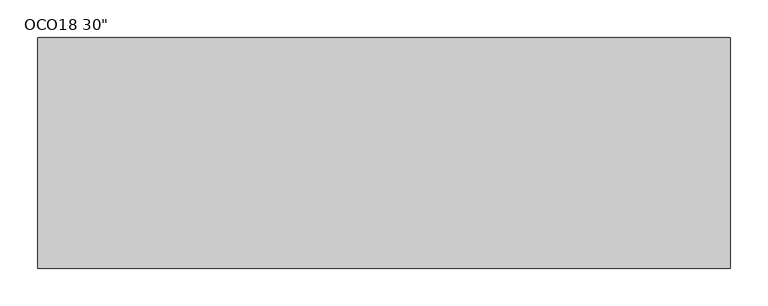
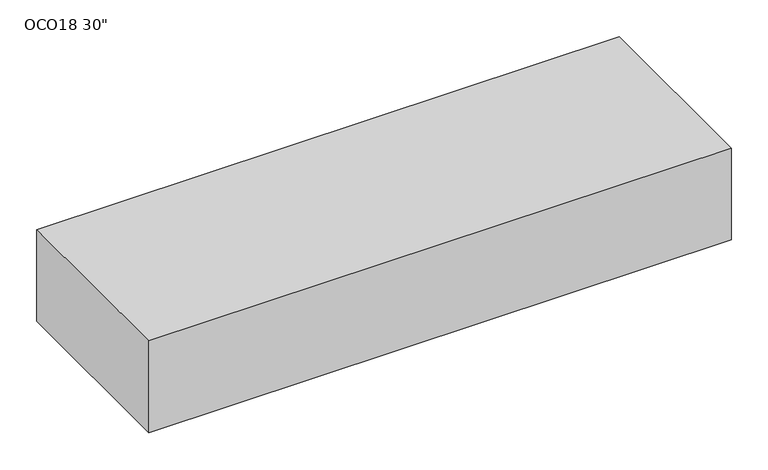
"""IFC4 building model written with IfcOpenShell, lengths in millimetres: furniture geometry."""

from ifc_helpers import new_model, si_unit, frame, origin, place, context, project, spatial, polyline, outline, extrude, faceted_brep, source, transform, mapped, element, save


def furniture_e9fbd180(model_context):
    return source(origin(), model_context, "Body", "SolidModel", [
        extrude(outline(polyline([(-125.8038372, 383.9486578), (-113.1038372, 383.9486578), (-113.1038372, 99.9612557), (-125.8038372, 99.9612557), (-125.8038372, 383.9486578)])), frame((0.0, 0.0, 1990.725), z_axis=(0.0, 0.0, 1.0), x_axis=(1.0, 0.0, 0.0)), (0.0, 0.0, 1.0), 133.35),
        extrude(outline(polyline([(172.6461628, 383.9486578), (185.3461628, 383.9486578), (185.3461628, 99.9612557), (172.6461628, 99.9612557), (172.6461628, 383.9486578)])), frame((0.0, 0.0, 1990.725), z_axis=(0.0, 0.0, 1.0), x_axis=(1.0, 0.0, 0.0)), (0.0, 0.0, 1.0), 133.35),
        extrude(outline(polyline([(-424.2538372, 383.9486578), (-411.5538372, 383.9486578), (-411.5538372, 99.9612557), (-424.2538372, 99.9612557), (-424.2538372, 383.9486578)])), frame((0.0, 0.0, 1990.725), z_axis=(0.0, 0.0, 1.0), x_axis=(1.0, 0.0, 0.0)), (0.0, 0.0, 1.0), 133.35),
        extrude(outline(polyline([(471.0961628, 383.9486578), (483.7961628, 383.9486578), (483.7961628, 99.9612557), (471.0961628, 99.9612557), (471.0961628, 383.9486578)])), frame((0.0, 0.0, 1990.725), z_axis=(0.0, 0.0, 1.0), x_axis=(1.0, 0.0, 0.0)), (0.0, 0.0, 1.0), 133.35),
        faceted_brep([(486.9711628, 385.7625, 1981.2), (-427.4288372, 385.7625, 1981.2), (-427.4288372, 385.7625, 2133.6), (486.9711628, 385.7625, 2133.6), (471.0961628, 385.7625, 1990.725), (471.0961628, 385.7625, 2124.075), (-411.5538372, 385.7625, 2124.075), (-411.5538372, 385.7625, 1990.725), (486.9711628, 80.9625, 1981.2), (486.9711628, 80.9625, 2133.6), (-427.4288372, 80.9625, 2133.6), (-427.4288372, 80.9625, 1981.2), (471.0961628, 99.9612557, 1990.725), (-411.5538372, 99.9612557, 1990.725), (-411.5538372, 99.9612557, 2124.075), (471.0961628, 99.9612557, 2124.075)], [[[0, 1, 2, 3], [4, 5, 6, 7]], [[8, 9, 10, 11]], [[1, 0, 8, 11]], [[2, 1, 11, 10]], [[3, 2, 10, 9]], [[0, 3, 9, 8]], [[12, 13, 14, 15]], [[12, 15, 5, 4]], [[15, 14, 6, 5]], [[14, 13, 7, 6]], [[13, 12, 4, 7]]]),
    ])


if __name__ == "__main__":
    model = new_model("IFC4")
    model_context = context("Model", 3, world=origin())
    ifc_project = project(units=[si_unit("LENGTHUNIT", "METRE", prefix="MILLI")], contexts=[model_context])
    site = spatial("IfcSite", under=ifc_project)
    building = spatial("IfcBuilding", under=site)
    placement = place(None, origin())
    furniture_shape = furniture_e9fbd180(model_context)
    element("IfcFurniture", 1, ObjectType="Accessories-Merillat-Wall-Open_Cube_Organizer : OCO18 30\"", at=placement, inside=building, context=model_context, shape_type="MappedRepresentation", body=[
        mapped(furniture_shape, transform((0.0, 0.0, 0.0), x_axis=(1.0, 0.0, 0.0), y_axis=(0.0, 1.0, 0.0), z_axis=(0.0, 0.0, 1.0))),
    ])
    save(model, "model.ifc")

# Revit data of these elements
# Type "Accessories-Merillat-Wall-Open_Cube_Organizer : OCO18 30\""
#   URL = "https://www.merillat.com/"
#   Product Page URL = "https://www.merillat.com/our-products/rooms/kitchen/"
#   Product Documentation Link = "http://merillatbusiness.com/wp-content/uploads/2014/07/Merillat_Classic_Catalog.pdf"
#   Model = "OCO18"
#   Manufacturer = "Merillat"
#   Finish = "Wood"
#   Description = "Open Cube Organizer 3 compartments"
#   Construction Type = "Wall Cabinet"
#   Assembly Code = "C1030410"
#   Depth = 1' - 0"
#   Height = 0' - 6"
#   Top Of Cabinet = 7' - 0"
#   Width = 3' - 0"
#   COBie.Type = no
#   Number of Compartments = 3
#   Actual Number of Compartments = 4
#   Cabinet Material = Wood - Merillat - Pecan(1)
# Element 1 (IfcFurniture, "Accessories-Merillat-Wall-Open_Cube_Organizer : OCO18 30\"")
#   Materials on its faces: "Wood - Merillat - Pecan(1)"
# Materials
#   "Wood - Merillat - Pecan(1)": class "Wood", colour RGB 108 67 43, transparency 0, Cost = 0
